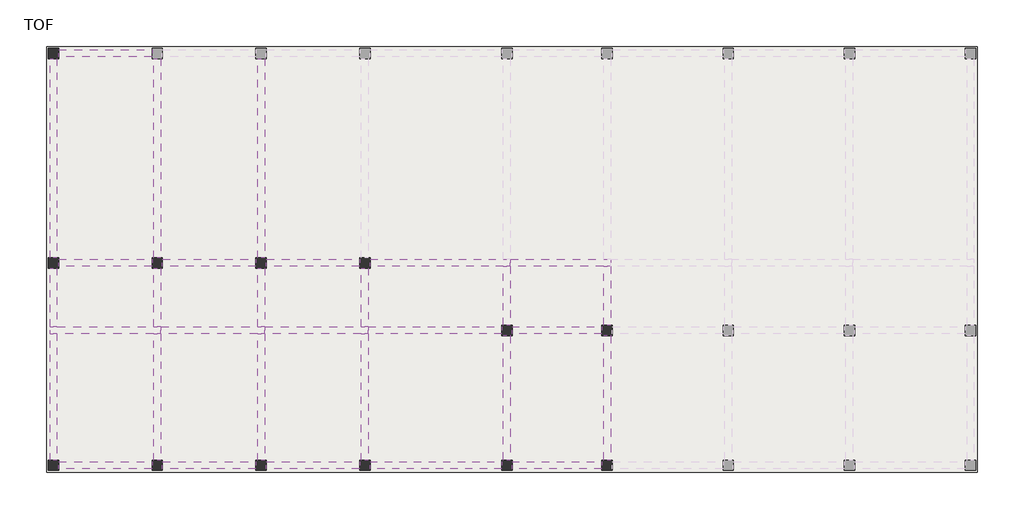
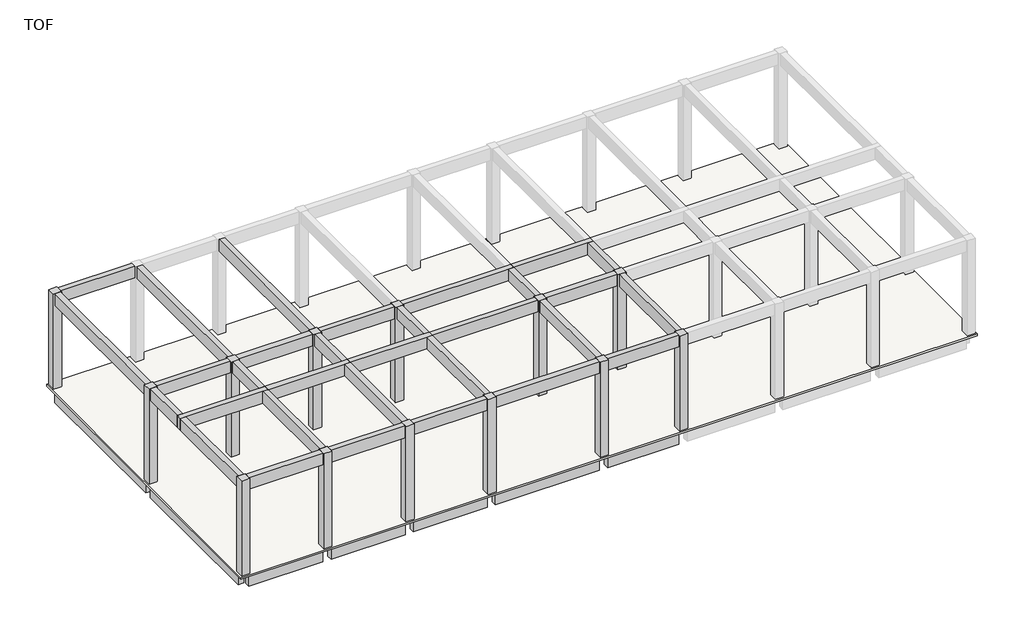
# One storey, part 1 of 2: 39 beams, 13 columns, 1 slab.
"""IFC4 building model written with IfcOpenShell, lengths in millimetres."""

from ifc_helpers import new_model, si_unit, frame, origin, origin_with_axes, place, context, project, spatial, polyline, outline, extrude, faceted_brep, element, save

model = new_model("IFC4")

# Units and contexts
model_context = context("Model", 3, world=origin())
ifc_project = project(units=[si_unit("LENGTHUNIT", "METRE", prefix="MILLI")], contexts=[model_context])

# Site, building, storey
site = spatial("IfcSite", under=ifc_project)
building = spatial("IfcBuilding", under=site)
storey = spatial("IfcBuildingStorey", under=building, Name="TOF", Elevation=150.0)

# Beams
placement = place(None, origin())
element("IfcBeam", 1, ObjectType="RC Beam_Rectangular : H_SB_ACB_B400xH900", at=placement, inside=storey, context=model_context, shape_type="SweptSolid", body=[
    extrude(outline(polyline([(124.7, 12616.5208589), (-275.3, 12616.5208589), (-275.3, 24116.5208589), (124.7, 24116.5208589), (124.7, 12616.5208589)])), frame((0.0, 0.0, -900.0), z_axis=(0.0, 0.0, 1.0), x_axis=(1.0, 0.0, 0.0)), (0.0, 0.0, 1.0), 900.0),
])
element("IfcBeam", 2, ObjectType="RC Beam_Rectangular : H_SB_ACB_B400xH900", at=placement, inside=storey, context=model_context, shape_type="SweptSolid", body=[
    extrude(outline(polyline([(124.7, 916.5208589), (-275.3, 916.5208589), (-275.3, 12016.5208589), (124.7, 12016.5208589), (124.7, 916.5208589)])), frame((0.0, 0.0, -900.0), z_axis=(0.0, 0.0, 1.0), x_axis=(1.0, 0.0, 0.0)), (0.0, 0.0, 1.0), 900.0),
])
element("IfcBeam", 3, ObjectType="RC Beam_Rectangular : H_SB_ACB_B400xH900", at=placement, inside=storey, context=model_context, shape_type="SweptSolid", body=[
    extrude(outline(polyline([(5624.7, 24616.5208589), (5624.7, 24216.5208589), (224.7, 24216.5208589), (224.7, 24616.5208589), (5624.7, 24616.5208589)])), frame((0.0, 0.0, -900.0), z_axis=(0.0, 0.0, 1.0), x_axis=(1.0, 0.0, 0.0)), (0.0, 0.0, 1.0), 900.0),
])
element("IfcBeam", 4, ObjectType="RC Beam_Rectangular : H_SB_ACB_B400xH900", at=placement, inside=storey, context=model_context, shape_type="SweptSolid", body=[
    extrude(outline(polyline([(224.7, 416.5208589), (224.7, 816.5208589), (5624.7, 816.5208589), (5624.7, 416.5208589), (224.7, 416.5208589)])), frame((0.0, 0.0, -900.0), z_axis=(0.0, 0.0, 1.0), x_axis=(1.0, 0.0, 0.0)), (0.0, 0.0, 1.0), 900.0),
])
element("IfcBeam", 5, ObjectType="RC Beam_Rectangular : H_SB_ACB_B400xH900", at=placement, inside=storey, context=model_context, shape_type="SweptSolid", body=[
    extrude(outline(polyline([(6224.7, 416.5208589), (6224.7, 816.5208589), (11624.7, 816.5208589), (11624.7, 416.5208589), (6224.7, 416.5208589)])), frame((0.0, 0.0, -900.0), z_axis=(0.0, 0.0, 1.0), x_axis=(1.0, 0.0, 0.0)), (0.0, 0.0, 1.0), 900.0),
])
element("IfcBeam", 6, ObjectType="RC Beam_Rectangular : H_SB_ACB_B400xH900", at=placement, inside=storey, context=model_context, shape_type="SweptSolid", body=[
    extrude(outline(polyline([(12224.7, 416.5208589), (12224.7, 816.5208589), (17624.7, 816.5208589), (17624.7, 416.5208589), (12224.7, 416.5208589)])), frame((0.0, 0.0, -900.0), z_axis=(0.0, 0.0, 1.0), x_axis=(1.0, 0.0, 0.0)), (0.0, 0.0, 1.0), 900.0),
])
element("IfcBeam", 7, ObjectType="RC Beam_Rectangular : H_SB_ACB_B400xH900", at=placement, inside=storey, context=model_context, shape_type="SweptSolid", body=[
    extrude(outline(polyline([(18224.7, 416.5208589), (18224.7, 816.5208589), (25824.7, 816.5208589), (25824.7, 416.5208589), (18224.7, 416.5208589)])), frame((0.0, 0.0, -900.0), z_axis=(0.0, 0.0, 1.0), x_axis=(1.0, 0.0, 0.0)), (0.0, 0.0, 1.0), 900.0),
])
element("IfcBeam", 8, ObjectType="RC Beam_Rectangular : H_SB_ACB_B400xH900", at=placement, inside=storey, context=model_context, shape_type="SweptSolid", body=[
    extrude(outline(polyline([(26424.7, 416.5208589), (26424.7, 816.5208589), (31624.7, 816.5208589), (31624.7, 416.5208589), (26424.7, 416.5208589)])), frame((0.0, 0.0, -900.0), z_axis=(0.0, 0.0, 1.0), x_axis=(1.0, 0.0, 0.0)), (0.0, 0.0, 1.0), 900.0),
])
element("IfcBeam", 9, ObjectType="RC Beam_Rectangular : H_SB_ACB_B400xH900", at=placement, inside=storey, context=model_context, shape_type="SweptSolid", body=[
    extrude(outline(polyline([(224.7, 12116.5208589), (224.7, 12516.5208589), (5624.7, 12516.5208589), (5624.7, 12116.5208589), (224.7, 12116.5208589)])), frame((0.0, 0.0, 6600.0), z_axis=(0.0, 0.0, 1.0), x_axis=(1.0, 0.0, 0.0)), (0.0, 0.0, 1.0), 900.0),
])
element("IfcBeam", 10, ObjectType="RC Beam_Rectangular : H_SB_ACB_B400xH900", at=placement, inside=storey, context=model_context, shape_type="SweptSolid", body=[
    extrude(outline(polyline([(6224.7, 12116.5208589), (6224.7, 12516.5208589), (11624.7, 12516.5208589), (11624.7, 12116.5208589), (6224.7, 12116.5208589)])), frame((0.0, 0.0, 6600.0), z_axis=(0.0, 0.0, 1.0), x_axis=(1.0, 0.0, 0.0)), (0.0, 0.0, 1.0), 900.0),
])
element("IfcBeam", 11, ObjectType="RC Beam_Rectangular : H_SB_ACB_B400xH900", at=placement, inside=storey, context=model_context, shape_type="SweptSolid", body=[
    extrude(outline(polyline([(12224.7, 12116.5208589), (12224.7, 12516.5208589), (17624.7, 12516.5208589), (17624.7, 12116.5208589), (12224.7, 12116.5208589)])), frame((0.0, 0.0, 6600.0), z_axis=(0.0, 0.0, 1.0), x_axis=(1.0, 0.0, 0.0)), (0.0, 0.0, 1.0), 900.0),
])
element("IfcBeam", 12, ObjectType="RC Beam_Rectangular : H_SB_ACB_B400xH900", at=placement, inside=storey, context=model_context, shape_type="Brep", body=[
    faceted_brep([(26324.7, 12116.5208589, 7500.0), (26324.7, 12516.5208589, 7500.0), (25924.7, 12516.5208589, 7500.0), (18224.7, 12516.5208589, 7500.0), (18224.7, 12116.5208589, 7500.0), (25924.7, 12116.5208589, 7500.0), (26324.7, 12116.5208589, 6600.0), (18224.7, 12116.5208589, 6600.0), (25924.7, 12116.5208589, 6600.0), (26324.7, 12516.5208589, 6600.0), (18224.7, 12516.5208589, 6600.0), (25924.7, 12516.5208589, 6600.0)], [[[0, 1, 2, 3, 4, 5]], [[6, 0, 5, 4, 7, 8]], [[9, 6, 8, 7, 10, 11]], [[1, 9, 11, 10, 3, 2]], [[4, 3, 10, 7]], [[1, 0, 6, 9]]]),
])
element("IfcBeam", 13, ObjectType="RC Beam_Rectangular : H_SB_ACB_B400xH900", at=placement, inside=storey, context=model_context, shape_type="Brep", body=[
    faceted_brep([(32124.7, 12116.5208589, 7500.0), (32124.7, 12516.5208589, 7500.0), (31724.7, 12516.5208589, 7500.0), (26324.7, 12516.5208589, 7500.0), (26324.7, 12116.5208589, 7500.0), (31724.7, 12116.5208589, 7500.0), (32124.7, 12116.5208589, 6600.0), (26324.7, 12116.5208589, 6600.0), (31724.7, 12116.5208589, 6600.0), (32124.7, 12516.5208589, 6600.0), (26324.7, 12516.5208589, 6600.0), (31724.7, 12516.5208589, 6600.0)], [[[0, 1, 2, 3, 4, 5]], [[6, 0, 5, 4, 7, 8]], [[9, 6, 8, 7, 10, 11]], [[1, 9, 11, 10, 3, 2]], [[1, 0, 6, 9]], [[4, 3, 10, 7]]]),
])
element("IfcBeam", 14, ObjectType="RC Beam_Rectangular : H_SB_ACB_B400xH900", at=placement, inside=storey, context=model_context, shape_type="SweptSolid", body=[
    extrude(outline(polyline([(224.7, 24216.5208589), (224.7, 24616.5208589), (5624.7, 24616.5208589), (5624.7, 24216.5208589), (224.7, 24216.5208589)])), frame((0.0, 0.0, 6600.0), z_axis=(0.0, 0.0, 1.0), x_axis=(1.0, 0.0, 0.0)), (0.0, 0.0, 1.0), 900.0),
])
element("IfcBeam", 15, ObjectType="RC Beam_Rectangular : H_SB_ACB_B400xH900", at=placement, inside=storey, context=model_context, shape_type="Brep", body=[
    faceted_brep([(-275.3, 8616.5208589, 7500.0), (-275.3, 8216.5208589, 7500.0), (124.7, 8216.5208589, 7500.0), (5724.7, 8216.5208589, 7500.0), (6124.7, 8216.5208589, 7500.0), (6124.7, 8616.5208589, 7500.0), (5724.7, 8616.5208589, 7500.0), (124.7, 8616.5208589, 7500.0), (-275.3, 8216.5208589, 6600.0), (124.7, 8216.5208589, 6600.0), (5724.7, 8216.5208589, 6600.0), (6124.7, 8216.5208589, 6600.0), (-275.3, 8616.5208589, 6600.0), (124.7, 8616.5208589, 6600.0), (5724.7, 8616.5208589, 6600.0), (6124.7, 8616.5208589, 6600.0)], [[[0, 1, 2, 3, 4, 5, 6, 7]], [[1, 8, 9, 10, 11, 4, 3, 2]], [[8, 12, 13, 14, 15, 11, 10, 9]], [[12, 0, 7, 6, 5, 15, 14, 13]], [[1, 0, 12, 8]], [[5, 4, 11, 15]]]),
])
element("IfcBeam", 16, ObjectType="RC Beam_Rectangular : H_SB_ACB_B400xH900", at=placement, inside=storey, context=model_context, shape_type="Brep", body=[
    faceted_brep([(12124.7, 8216.5208589, 7500.0), (12124.7, 8616.5208589, 7500.0), (11724.7, 8616.5208589, 7500.0), (6124.7, 8616.5208589, 7500.0), (6124.7, 8216.5208589, 7500.0), (11724.7, 8216.5208589, 7500.0), (12124.7, 8216.5208589, 6600.0), (6124.7, 8216.5208589, 6600.0), (11724.7, 8216.5208589, 6600.0), (12124.7, 8616.5208589, 6600.0), (6124.7, 8616.5208589, 6600.0), (11724.7, 8616.5208589, 6600.0)], [[[0, 1, 2, 3, 4, 5]], [[6, 0, 5, 4, 7, 8]], [[9, 6, 8, 7, 10, 11]], [[1, 9, 11, 10, 3, 2]], [[1, 0, 6, 9]], [[4, 3, 10, 7]]]),
])
element("IfcBeam", 17, ObjectType="RC Beam_Rectangular : H_SB_ACB_B400xH900", at=placement, inside=storey, context=model_context, shape_type="Brep", body=[
    faceted_brep([(18124.7, 8216.5208589, 7500.0), (18124.7, 8616.5208589, 7500.0), (17724.7, 8616.5208589, 7500.0), (12124.7, 8616.5208589, 7500.0), (12124.7, 8216.5208589, 7500.0), (17724.7, 8216.5208589, 7500.0), (18124.7, 8216.5208589, 6600.0), (12124.7, 8216.5208589, 6600.0), (17724.7, 8216.5208589, 6600.0), (18124.7, 8616.5208589, 6600.0), (12124.7, 8616.5208589, 6600.0), (17724.7, 8616.5208589, 6600.0)], [[[0, 1, 2, 3, 4, 5]], [[6, 0, 5, 4, 7, 8]], [[9, 6, 8, 7, 10, 11]], [[1, 9, 11, 10, 3, 2]], [[1, 0, 6, 9]], [[4, 3, 10, 7]]]),
])
element("IfcBeam", 18, ObjectType="RC Beam_Rectangular : H_SB_ACB_B400xH900", at=placement, inside=storey, context=model_context, shape_type="SweptSolid", body=[
    extrude(outline(polyline([(18124.7, 8216.5208589), (18124.7, 8616.5208589), (25824.7, 8616.5208589), (25824.7, 8216.5208589), (18124.7, 8216.5208589)])), frame((0.0, 0.0, 6600.0), z_axis=(0.0, 0.0, 1.0), x_axis=(1.0, 0.0, 0.0)), (0.0, 0.0, 1.0), 900.0),
])
element("IfcBeam", 19, ObjectType="RC Beam_Rectangular : H_SB_ACB_B400xH900", at=placement, inside=storey, context=model_context, shape_type="SweptSolid", body=[
    extrude(outline(polyline([(26424.7, 8216.5208589), (26424.7, 8616.5208589), (31624.7, 8616.5208589), (31624.7, 8216.5208589), (26424.7, 8216.5208589)])), frame((0.0, 0.0, 6600.0), z_axis=(0.0, 0.0, 1.0), x_axis=(1.0, 0.0, 0.0)), (0.0, 0.0, 1.0), 900.0),
])
element("IfcBeam", 20, ObjectType="RC Beam_Rectangular : H_SB_ACB_B400xH900", at=placement, inside=storey, context=model_context, shape_type="SweptSolid", body=[
    extrude(outline(polyline([(224.7, 416.5208589), (224.7, 816.5208589), (5624.7, 816.5208589), (5624.7, 416.5208589), (224.7, 416.5208589)])), frame((0.0, 0.0, 6600.0), z_axis=(0.0, 0.0, 1.0), x_axis=(1.0, 0.0, 0.0)), (0.0, 0.0, 1.0), 900.0),
])
element("IfcBeam", 21, ObjectType="RC Beam_Rectangular : H_SB_ACB_B400xH900", at=placement, inside=storey, context=model_context, shape_type="SweptSolid", body=[
    extrude(outline(polyline([(6224.7, 416.5208589), (6224.7, 816.5208589), (11624.7, 816.5208589), (11624.7, 416.5208589), (6224.7, 416.5208589)])), frame((0.0, 0.0, 6600.0), z_axis=(0.0, 0.0, 1.0), x_axis=(1.0, 0.0, 0.0)), (0.0, 0.0, 1.0), 900.0),
])
element("IfcBeam", 22, ObjectType="RC Beam_Rectangular : H_SB_ACB_B400xH900", at=placement, inside=storey, context=model_context, shape_type="SweptSolid", body=[
    extrude(outline(polyline([(12224.7, 416.5208589), (12224.7, 816.5208589), (17624.7, 816.5208589), (17624.7, 416.5208589), (12224.7, 416.5208589)])), frame((0.0, 0.0, 6600.0), z_axis=(0.0, 0.0, 1.0), x_axis=(1.0, 0.0, 0.0)), (0.0, 0.0, 1.0), 900.0),
])
element("IfcBeam", 23, ObjectType="RC Beam_Rectangular : H_SB_ACB_B400xH900", at=placement, inside=storey, context=model_context, shape_type="SweptSolid", body=[
    extrude(outline(polyline([(18224.7, 416.5208589), (18224.7, 816.5208589), (25824.7, 816.5208589), (25824.7, 416.5208589), (18224.7, 416.5208589)])), frame((0.0, 0.0, 6600.0), z_axis=(0.0, 0.0, 1.0), x_axis=(1.0, 0.0, 0.0)), (0.0, 0.0, 1.0), 900.0),
])
element("IfcBeam", 24, ObjectType="RC Beam_Rectangular : H_SB_ACB_B400xH900", at=placement, inside=storey, context=model_context, shape_type="SweptSolid", body=[
    extrude(outline(polyline([(26424.7, 416.5208589), (26424.7, 816.5208589), (31624.7, 816.5208589), (31624.7, 416.5208589), (26424.7, 416.5208589)])), frame((0.0, 0.0, 6600.0), z_axis=(0.0, 0.0, 1.0), x_axis=(1.0, 0.0, 0.0)), (0.0, 0.0, 1.0), 900.0),
])
element("IfcBeam", 25, ObjectType="RC Beam_Rectangular : H_SB_ACB_B400xH900", at=placement, inside=storey, context=model_context, shape_type="SweptSolid", body=[
    extrude(outline(polyline([(-275.3, 8216.5208589), (124.7, 8216.5208589), (124.7, 916.5208589), (-275.3, 916.5208589), (-275.3, 8216.5208589)])), frame((0.0, 0.0, 6600.0), z_axis=(0.0, 0.0, 1.0), x_axis=(1.0, 0.0, 0.0)), (0.0, 0.0, 1.0), 900.0),
])
element("IfcBeam", 26, ObjectType="RC Beam_Rectangular : H_SB_ACB_B400xH900", at=placement, inside=storey, context=model_context, shape_type="SweptSolid", body=[
    extrude(outline(polyline([(124.7, 8616.5208589), (-275.3, 8616.5208589), (-275.3, 12016.5208589), (124.7, 12016.5208589), (124.7, 8616.5208589)])), frame((0.0, 0.0, 6600.0), z_axis=(0.0, 0.0, 1.0), x_axis=(1.0, 0.0, 0.0)), (0.0, 0.0, 1.0), 900.0),
])
element("IfcBeam", 27, ObjectType="RC Beam_Rectangular : H_SB_ACB_B400xH900", at=placement, inside=storey, context=model_context, shape_type="SweptSolid", body=[
    extrude(outline(polyline([(124.7, 12616.5208589), (-275.3, 12616.5208589), (-275.3, 24116.5208589), (124.7, 24116.5208589), (124.7, 12616.5208589)])), frame((0.0, 0.0, 6600.0), z_axis=(0.0, 0.0, 1.0), x_axis=(1.0, 0.0, 0.0)), (0.0, 0.0, 1.0), 900.0),
])
element("IfcBeam", 28, ObjectType="RC Beam_Rectangular : H_SB_ACB_B400xH900", at=placement, inside=storey, context=model_context, shape_type="SweptSolid", body=[
    extrude(outline(polyline([(5724.7, 8216.5208589), (6124.7, 8216.5208589), (6124.7, 916.5208589), (5724.7, 916.5208589), (5724.7, 8216.5208589)])), frame((0.0, 0.0, 6600.0), z_axis=(0.0, 0.0, 1.0), x_axis=(1.0, 0.0, 0.0)), (0.0, 0.0, 1.0), 900.0),
])
element("IfcBeam", 29, ObjectType="RC Beam_Rectangular : H_SB_ACB_B400xH900", at=placement, inside=storey, context=model_context, shape_type="SweptSolid", body=[
    extrude(outline(polyline([(6124.7, 8616.5208589), (5724.7, 8616.5208589), (5724.7, 12016.5208589), (6124.7, 12016.5208589), (6124.7, 8616.5208589)])), frame((0.0, 0.0, 6600.0), z_axis=(0.0, 0.0, 1.0), x_axis=(1.0, 0.0, 0.0)), (0.0, 0.0, 1.0), 900.0),
])
element("IfcBeam", 30, ObjectType="RC Beam_Rectangular : H_SB_ACB_B400xH900", at=placement, inside=storey, context=model_context, shape_type="SweptSolid", body=[
    extrude(outline(polyline([(6124.7, 12616.5208589), (5724.7, 12616.5208589), (5724.7, 24116.5208589), (6124.7, 24116.5208589), (6124.7, 12616.5208589)])), frame((0.0, 0.0, 6600.0), z_axis=(0.0, 0.0, 1.0), x_axis=(1.0, 0.0, 0.0)), (0.0, 0.0, 1.0), 900.0),
])
element("IfcBeam", 31, ObjectType="RC Beam_Rectangular : H_SB_ACB_B400xH900", at=placement, inside=storey, context=model_context, shape_type="SweptSolid", body=[
    extrude(outline(polyline([(11724.7, 8216.5208589), (12124.7, 8216.5208589), (12124.7, 916.5208589), (11724.7, 916.5208589), (11724.7, 8216.5208589)])), frame((0.0, 0.0, 6600.0), z_axis=(0.0, 0.0, 1.0), x_axis=(1.0, 0.0, 0.0)), (0.0, 0.0, 1.0), 900.0),
])
element("IfcBeam", 32, ObjectType="RC Beam_Rectangular : H_SB_ACB_B400xH900", at=placement, inside=storey, context=model_context, shape_type="SweptSolid", body=[
    extrude(outline(polyline([(12124.7, 8616.5208589), (11724.7, 8616.5208589), (11724.7, 12016.5208589), (12124.7, 12016.5208589), (12124.7, 8616.5208589)])), frame((0.0, 0.0, 6600.0), z_axis=(0.0, 0.0, 1.0), x_axis=(1.0, 0.0, 0.0)), (0.0, 0.0, 1.0), 900.0),
])
element("IfcBeam", 33, ObjectType="RC Beam_Rectangular : H_SB_ACB_B400xH900", at=placement, inside=storey, context=model_context, shape_type="SweptSolid", body=[
    extrude(outline(polyline([(12124.7, 12616.5208589), (11724.7, 12616.5208589), (11724.7, 24116.5208589), (12124.7, 24116.5208589), (12124.7, 12616.5208589)])), frame((0.0, 0.0, 6600.0), z_axis=(0.0, 0.0, 1.0), x_axis=(1.0, 0.0, 0.0)), (0.0, 0.0, 1.0), 900.0),
])
element("IfcBeam", 34, ObjectType="RC Beam_Rectangular : H_SB_ACB_B400xH900", at=placement, inside=storey, context=model_context, shape_type="SweptSolid", body=[
    extrude(outline(polyline([(17724.7, 8216.5208589), (18124.7, 8216.5208589), (18124.7, 916.5208589), (17724.7, 916.5208589), (17724.7, 8216.5208589)])), frame((0.0, 0.0, 6600.0), z_axis=(0.0, 0.0, 1.0), x_axis=(1.0, 0.0, 0.0)), (0.0, 0.0, 1.0), 900.0),
])
element("IfcBeam", 35, ObjectType="RC Beam_Rectangular : H_SB_ACB_B400xH900", at=placement, inside=storey, context=model_context, shape_type="SweptSolid", body=[
    extrude(outline(polyline([(18124.7, 8616.5208589), (17724.7, 8616.5208589), (17724.7, 12016.5208589), (18124.7, 12016.5208589), (18124.7, 8616.5208589)])), frame((0.0, 0.0, 6600.0), z_axis=(0.0, 0.0, 1.0), x_axis=(1.0, 0.0, 0.0)), (0.0, 0.0, 1.0), 900.0),
])
element("IfcBeam", 36, ObjectType="RC Beam_Rectangular : H_SB_ACB_B400xH900", at=placement, inside=storey, context=model_context, shape_type="SweptSolid", body=[
    extrude(outline(polyline([(25924.7, 8116.5208589), (26324.7, 8116.5208589), (26324.7, 916.5208589), (25924.7, 916.5208589), (25924.7, 8116.5208589)])), frame((0.0, 0.0, 6600.0), z_axis=(0.0, 0.0, 1.0), x_axis=(1.0, 0.0, 0.0)), (0.0, 0.0, 1.0), 900.0),
])
element("IfcBeam", 37, ObjectType="RC Beam_Rectangular : H_SB_ACB_B400xH900", at=placement, inside=storey, context=model_context, shape_type="SweptSolid", body=[
    extrude(outline(polyline([(25924.7, 12116.5208589), (26324.7, 12116.5208589), (26324.7, 8716.5208589), (25924.7, 8716.5208589), (25924.7, 12116.5208589)])), frame((0.0, 0.0, 6600.0), z_axis=(0.0, 0.0, 1.0), x_axis=(1.0, 0.0, 0.0)), (0.0, 0.0, 1.0), 900.0),
])
element("IfcBeam", 38, ObjectType="RC Beam_Rectangular : H_SB_ACB_B400xH900", at=placement, inside=storey, context=model_context, shape_type="SweptSolid", body=[
    extrude(outline(polyline([(31724.7, 8116.5208589), (32124.7, 8116.5208589), (32124.7, 916.5208589), (31724.7, 916.5208589), (31724.7, 8116.5208589)])), frame((0.0, 0.0, 6600.0), z_axis=(0.0, 0.0, 1.0), x_axis=(1.0, 0.0, 0.0)), (0.0, 0.0, 1.0), 900.0),
])
element("IfcBeam", 39, ObjectType="RC Beam_Rectangular : H_SB_ACB_B400xH900", at=placement, inside=storey, context=model_context, shape_type="SweptSolid", body=[
    extrude(outline(polyline([(31724.7, 12116.5208589), (32124.7, 12116.5208589), (32124.7, 8716.5208589), (31724.7, 8716.5208589), (31724.7, 12116.5208589)])), frame((0.0, 0.0, 6600.0), z_axis=(0.0, 0.0, 1.0), x_axis=(1.0, 0.0, 0.0)), (0.0, 0.0, 1.0), 900.0),
])

# Columns
element("IfcColumn", 40, ObjectType="RC_Column_Rectangular : H_SC_ACC_W600xL600", at=placement, inside=storey, context=model_context, shape_type="Brep", body=[
    faceted_brep([(224.7, 12616.5208589, 7500.0), (224.7, 12516.5208589, 7500.0), (224.7, 12116.5208589, 7500.0), (224.7, 12016.5208589, 7500.0), (224.7, 12016.5208589, 150.0), (224.7, 12616.5208589, 150.0), (124.7, 12016.5208589, 7500.0), (-275.3, 12016.5208589, 7500.0), (-375.3, 12016.5208589, 7500.0), (-375.3, 12016.5208589, 150.0), (-375.3, 12616.5208589, 7500.0), (-375.3, 12616.5208589, 150.0), (-275.3, 12616.5208589, 7500.0), (124.7, 12616.5208589, 7500.0)], [[[0, 1, 2, 3, 4, 5]], [[3, 6, 7, 8, 9, 4]], [[8, 10, 11, 9]], [[10, 12, 13, 0, 5, 11]], [[3, 2, 1, 0, 13, 12, 10, 8, 7, 6]], [[5, 4, 9, 11]]]),
])
element("IfcColumn", 41, ObjectType="RC_Column_Rectangular : H_SC_ACC_W600xL600", at=placement, inside=storey, context=model_context, shape_type="Brep", body=[
    faceted_brep([(6224.7, 12616.5208589, 7500.0), (6224.7, 12516.5208589, 7500.0), (6224.7, 12116.5208589, 7500.0), (6224.7, 12016.5208589, 7500.0), (6224.7, 12016.5208589, 150.0), (6224.7, 12616.5208589, 150.0), (6124.7, 12016.5208589, 7500.0), (5724.7, 12016.5208589, 7500.0), (5624.7, 12016.5208589, 7500.0), (5624.7, 12016.5208589, 150.0), (5624.7, 12116.5208589, 7500.0), (5624.7, 12516.5208589, 7500.0), (5624.7, 12616.5208589, 7500.0), (5624.7, 12616.5208589, 150.0), (5724.7, 12616.5208589, 7500.0), (6124.7, 12616.5208589, 7500.0)], [[[0, 1, 2, 3, 4, 5]], [[3, 6, 7, 8, 9, 4]], [[8, 10, 11, 12, 13, 9]], [[12, 14, 15, 0, 5, 13]], [[3, 2, 1, 0, 15, 14, 12, 11, 10, 8, 7, 6]], [[5, 4, 9, 13]]]),
])
element("IfcColumn", 42, ObjectType="RC_Column_Rectangular : H_SC_ACC_W600xL600", at=placement, inside=storey, context=model_context, shape_type="Brep", body=[
    faceted_brep([(12224.7, 12616.5208589, 7500.0), (12224.7, 12516.5208589, 7500.0), (12224.7, 12116.5208589, 7500.0), (12224.7, 12016.5208589, 7500.0), (12224.7, 12016.5208589, 150.0), (12224.7, 12616.5208589, 150.0), (12124.7, 12016.5208589, 7500.0), (11724.7, 12016.5208589, 7500.0), (11624.7, 12016.5208589, 7500.0), (11624.7, 12016.5208589, 150.0), (11624.7, 12116.5208589, 7500.0), (11624.7, 12516.5208589, 7500.0), (11624.7, 12616.5208589, 7500.0), (11624.7, 12616.5208589, 150.0), (11724.7, 12616.5208589, 7500.0), (12124.7, 12616.5208589, 7500.0)], [[[0, 1, 2, 3, 4, 5]], [[3, 6, 7, 8, 9, 4]], [[8, 10, 11, 12, 13, 9]], [[12, 14, 15, 0, 5, 13]], [[3, 2, 1, 0, 15, 14, 12, 11, 10, 8, 7, 6]], [[5, 4, 9, 13]]]),
])
element("IfcColumn", 43, ObjectType="RC_Column_Rectangular : H_SC_ACC_W600xL600", at=placement, inside=storey, context=model_context, shape_type="Brep", body=[
    faceted_brep([(18224.7, 12616.5208589, 7500.0), (18224.7, 12516.5208589, 7500.0), (18224.7, 12116.5208589, 7500.0), (18224.7, 12016.5208589, 7500.0), (18224.7, 12016.5208589, 150.0), (18224.7, 12616.5208589, 150.0), (18124.7, 12016.5208589, 7500.0), (17724.7, 12016.5208589, 7500.0), (17624.7, 12016.5208589, 7500.0), (17624.7, 12016.5208589, 150.0), (17624.7, 12116.5208589, 7500.0), (17624.7, 12516.5208589, 7500.0), (17624.7, 12616.5208589, 7500.0), (17624.7, 12616.5208589, 150.0), (17724.7, 12616.5208589, 7500.0), (18124.7, 12616.5208589, 7500.0)], [[[0, 1, 2, 3, 4, 5]], [[3, 6, 7, 8, 9, 4]], [[8, 10, 11, 12, 13, 9]], [[12, 14, 15, 0, 5, 13]], [[3, 2, 1, 0, 15, 14, 12, 11, 10, 8, 7, 6]], [[5, 4, 9, 13]]]),
])
element("IfcColumn", 44, ObjectType="RC_Column_Rectangular : H_SC_ACC_W600xL600", at=placement, inside=storey, context=model_context, shape_type="Brep", body=[
    faceted_brep([(224.7, 24716.5208589, 7500.0), (224.7, 24616.5208589, 7500.0), (224.7, 24216.5208589, 7500.0), (224.7, 24116.5208589, 7500.0), (224.7, 24116.5208589, 150.0), (224.7, 24716.5208589, 150.0), (124.7, 24116.5208589, 7500.0), (-275.3, 24116.5208589, 7500.0), (-375.3, 24116.5208589, 7500.0), (-375.3, 24116.5208589, 150.0), (-375.3, 24716.5208589, 7500.0), (-375.3, 24716.5208589, 150.0)], [[[0, 1, 2, 3, 4, 5]], [[3, 6, 7, 8, 9, 4]], [[8, 10, 11, 9]], [[10, 0, 5, 11]], [[3, 2, 1, 0, 10, 8, 7, 6]], [[5, 4, 9, 11]]]),
])
element("IfcColumn", 45, ObjectType="RC_Column_Rectangular : H_SC_ACC_W600xL600", at=placement, inside=storey, context=model_context, shape_type="Brep", body=[
    faceted_brep([(26424.7, 8716.5208589, 7500.0), (26424.7, 8616.5208589, 7500.0), (26424.7, 8216.5208589, 7500.0), (26424.7, 8116.5208589, 7500.0), (26424.7, 8116.5208589, 150.0), (26424.7, 8716.5208589, 150.0), (26324.7, 8116.5208589, 7500.0), (25924.7, 8116.5208589, 7500.0), (25824.7, 8116.5208589, 7500.0), (25824.7, 8116.5208589, 150.0), (25824.7, 8216.5208589, 7500.0), (25824.7, 8616.5208589, 7500.0), (25824.7, 8716.5208589, 7500.0), (25824.7, 8716.5208589, 150.0), (25924.7, 8716.5208589, 7500.0), (26324.7, 8716.5208589, 7500.0)], [[[0, 1, 2, 3, 4, 5]], [[3, 6, 7, 8, 9, 4]], [[8, 10, 11, 12, 13, 9]], [[12, 14, 15, 0, 5, 13]], [[3, 2, 1, 0, 15, 14, 12, 11, 10, 8, 7, 6]], [[5, 4, 9, 13]]]),
])
element("IfcColumn", 46, ObjectType="RC_Column_Rectangular : H_SC_ACC_W600xL600", at=placement, inside=storey, context=model_context, shape_type="Brep", body=[
    faceted_brep([(32224.7, 8716.5208589, 7500.0), (32224.7, 8616.5208589, 7500.0), (32224.7, 8216.5208589, 7500.0), (32224.7, 8116.5208589, 7500.0), (32224.7, 8116.5208589, 150.0), (32224.7, 8716.5208589, 150.0), (32124.7, 8116.5208589, 7500.0), (31724.7, 8116.5208589, 7500.0), (31624.7, 8116.5208589, 7500.0), (31624.7, 8116.5208589, 150.0), (31624.7, 8216.5208589, 7500.0), (31624.7, 8616.5208589, 7500.0), (31624.7, 8716.5208589, 7500.0), (31624.7, 8716.5208589, 150.0), (31724.7, 8716.5208589, 7500.0), (32124.7, 8716.5208589, 7500.0)], [[[0, 1, 2, 3, 4, 5]], [[3, 6, 7, 8, 9, 4]], [[8, 10, 11, 12, 13, 9]], [[12, 14, 15, 0, 5, 13]], [[3, 2, 1, 0, 15, 14, 12, 11, 10, 8, 7, 6]], [[5, 4, 9, 13]]]),
])
element("IfcColumn", 47, ObjectType="RC_Column_Rectangular : H_SC_ACC_W600xL600", at=placement, inside=storey, context=model_context, shape_type="Brep", body=[
    faceted_brep([(224.7, 916.5208589, 7500.0), (224.7, 816.5208589, 7500.0), (224.7, 416.5208589, 7500.0), (224.7, 316.5208589, 7500.0), (224.7, 316.5208589, 150.0), (224.7, 916.5208589, 150.0), (-375.3, 316.5208589, 7500.0), (-375.3, 316.5208589, 150.0), (-375.3, 916.5208589, 7500.0), (-375.3, 916.5208589, 150.0), (-275.3, 916.5208589, 7500.0), (124.7, 916.5208589, 7500.0)], [[[0, 1, 2, 3, 4, 5]], [[3, 6, 7, 4]], [[6, 8, 9, 7]], [[8, 10, 11, 0, 5, 9]], [[3, 2, 1, 0, 11, 10, 8, 6]], [[5, 4, 7, 9]]]),
])
element("IfcColumn", 48, ObjectType="RC_Column_Rectangular : H_SC_ACC_W600xL600", at=placement, inside=storey, context=model_context, shape_type="Brep", body=[
    faceted_brep([(6224.7, 916.5208589, 7500.0), (6224.7, 816.5208589, 7500.0), (6224.7, 416.5208589, 7500.0), (6224.7, 316.5208589, 7500.0), (6224.7, 316.5208589, 150.0), (6224.7, 916.5208589, 150.0), (5624.7, 316.5208589, 7500.0), (5624.7, 316.5208589, 150.0), (5624.7, 416.5208589, 7500.0), (5624.7, 816.5208589, 7500.0), (5624.7, 916.5208589, 7500.0), (5624.7, 916.5208589, 150.0), (5724.7, 916.5208589, 7500.0), (6124.7, 916.5208589, 7500.0)], [[[0, 1, 2, 3, 4, 5]], [[3, 6, 7, 4]], [[6, 8, 9, 10, 11, 7]], [[10, 12, 13, 0, 5, 11]], [[3, 2, 1, 0, 13, 12, 10, 9, 8, 6]], [[5, 4, 7, 11]]]),
])
element("IfcColumn", 49, ObjectType="RC_Column_Rectangular : H_SC_ACC_W600xL600", at=placement, inside=storey, context=model_context, shape_type="Brep", body=[
    faceted_brep([(12224.7, 916.5208589, 7500.0), (12224.7, 816.5208589, 7500.0), (12224.7, 416.5208589, 7500.0), (12224.7, 316.5208589, 7500.0), (12224.7, 316.5208589, 150.0), (12224.7, 916.5208589, 150.0), (11624.7, 316.5208589, 7500.0), (11624.7, 316.5208589, 150.0), (11624.7, 416.5208589, 7500.0), (11624.7, 816.5208589, 7500.0), (11624.7, 916.5208589, 7500.0), (11624.7, 916.5208589, 150.0), (11724.7, 916.5208589, 7500.0), (12124.7, 916.5208589, 7500.0)], [[[0, 1, 2, 3, 4, 5]], [[3, 6, 7, 4]], [[6, 8, 9, 10, 11, 7]], [[10, 12, 13, 0, 5, 11]], [[3, 2, 1, 0, 13, 12, 10, 9, 8, 6]], [[5, 4, 7, 11]]]),
])
element("IfcColumn", 50, ObjectType="RC_Column_Rectangular : H_SC_ACC_W600xL600", at=placement, inside=storey, context=model_context, shape_type="Brep", body=[
    faceted_brep([(18224.7, 916.5208589, 7500.0), (18224.7, 816.5208589, 7500.0), (18224.7, 416.5208589, 7500.0), (18224.7, 316.5208589, 7500.0), (18224.7, 316.5208589, 150.0), (18224.7, 916.5208589, 150.0), (17624.7, 316.5208589, 7500.0), (17624.7, 316.5208589, 150.0), (17624.7, 416.5208589, 7500.0), (17624.7, 816.5208589, 7500.0), (17624.7, 916.5208589, 7500.0), (17624.7, 916.5208589, 150.0), (17724.7, 916.5208589, 7500.0), (18124.7, 916.5208589, 7500.0)], [[[0, 1, 2, 3, 4, 5]], [[3, 6, 7, 4]], [[6, 8, 9, 10, 11, 7]], [[10, 12, 13, 0, 5, 11]], [[3, 2, 1, 0, 13, 12, 10, 9, 8, 6]], [[5, 4, 7, 11]]]),
])
element("IfcColumn", 51, ObjectType="RC_Column_Rectangular : H_SC_ACC_W600xL600", at=placement, inside=storey, context=model_context, shape_type="Brep", body=[
    faceted_brep([(26424.7, 916.5208589, 7500.0), (26424.7, 816.5208589, 7500.0), (26424.7, 416.5208589, 7500.0), (26424.7, 316.5208589, 7500.0), (26424.7, 316.5208589, 150.0), (26424.7, 916.5208589, 150.0), (25824.7, 316.5208589, 7500.0), (25824.7, 316.5208589, 150.0), (25824.7, 416.5208589, 7500.0), (25824.7, 816.5208589, 7500.0), (25824.7, 916.5208589, 7500.0), (25824.7, 916.5208589, 150.0), (25924.7, 916.5208589, 7500.0), (26324.7, 916.5208589, 7500.0)], [[[0, 1, 2, 3, 4, 5]], [[3, 6, 7, 4]], [[6, 8, 9, 10, 11, 7]], [[10, 12, 13, 0, 5, 11]], [[3, 2, 1, 0, 13, 12, 10, 9, 8, 6]], [[5, 4, 7, 11]]]),
])
element("IfcColumn", 52, ObjectType="RC_Column_Rectangular : H_SC_ACC_W600xL600", at=placement, inside=storey, context=model_context, shape_type="Brep", body=[
    faceted_brep([(32224.7, 916.5208589, 7500.0), (32224.7, 816.5208589, 7500.0), (32224.7, 416.5208589, 7500.0), (32224.7, 316.5208589, 7500.0), (32224.7, 316.5208589, 150.0), (32224.7, 916.5208589, 150.0), (31624.7, 316.5208589, 7500.0), (31624.7, 316.5208589, 150.0), (31624.7, 416.5208589, 7500.0), (31624.7, 816.5208589, 7500.0), (31624.7, 916.5208589, 7500.0), (31624.7, 916.5208589, 150.0), (31724.7, 916.5208589, 7500.0), (32124.7, 916.5208589, 7500.0)], [[[0, 1, 2, 3, 4, 5]], [[3, 6, 7, 4]], [[6, 8, 9, 10, 11, 7]], [[10, 12, 13, 0, 5, 11]], [[3, 2, 1, 0, 13, 12, 10, 9, 8, 6]], [[5, 4, 7, 11]]]),
])

# Slab
element("IfcSlab", 53, ObjectType="H_FL_AMF_RC Slab_T150", at=placement, inside=storey, context=model_context, shape_type="SweptSolid", body=[
    extrude(outline(polyline([(53324.7, 216.5208589), (-475.3, 216.5208589), (-475.3, 24816.5208589), (53324.7, 24816.5208589), (53324.7, 216.5208589)])), origin_with_axes(), (0.0, 0.0, 1.0), 150.0),
])

save(model, "model.ifc")

# Revit data of these elements
# Project information
#   Project Status = "Project Status"
#   Client Name = "현대엔지니어링"
#   Project Address = "서울시 종로구 율곡로 75(계동)"
#   Project Number = "-"
# Grids (mm)
#   "Y1": line (-3935.398, 24416.521) -> (58968.688, 24416.521)
#   "X1": line (-75.3, 29394.337) -> (-75.3, -4379.638)
#   "X2": line (5924.7, 29394.337) -> (5924.7, -4379.638)
#   "Y3": line (-3935.398, 8416.521) -> (58968.688, 8416.521)
#   "Y4": line (-3935.398, 616.521) -> (58968.688, 616.521)
#   "X3": line (11924.7, 29394.337) -> (11924.7, -4379.638)
#   "X4": line (17924.7, 29394.337) -> (17924.7, -4379.638)
#   "X5": line (26124.7, 29394.337) -> (26124.7, -4379.638)
#   "X6": line (31924.7, 29394.337) -> (31924.7, -4379.638)
#   "X7": line (38924.7, 29394.337) -> (38924.7, -4379.638)
#   "X8": line (45924.7, 29394.337) -> (45924.7, -4379.638)
#   "X9": line (52924.7, 29394.337) -> (52924.7, -4379.638)
#   "X15": line (43724.7, 27041.858) -> (43724.7, 9156.488)
#   "X16": line (36324.7, 27041.858) -> (36324.7, 9156.488)
#   "X17": line (34685.051, 10966.521) -> (55094.626, 10966.521)
#   "X18": line (34685.051, 18666.521) -> (55094.626, 18666.521)
#   "Y2": line (-3935.398, 12316.521) -> (58968.688, 12316.521)
# Type "RC Beam_Rectangular : H_SB_ACB_B400xH900"
#   중앙부 하부근 = ""
#   중앙부 상부근 = ""
#   중앙부 보조근 = ""
#   중앙부 늑근 = ""
#   외단부 하부근 = ""
#   외단부 상부근 = ""
#   외단부 보조근 = ""
#   외단부 늑근 = ""
#   부호 = "TG3"
#   내단부 하부근 = ""
#   내단부 상부근 = ""
#   내단부 보조근 = ""
#   내단부 늑근 = ""
#   ALL 하부근 = "3-D20"
#   ALL 상부근 = "3-D20"
#   ALL 보조근 = ""
#   ALL 늑근 = "2-D10 @120"
#   Width = 400.000 mm
#   Height = 900.000 mm
#   Length [instance default] = 1524.000 mm
#   b = 400.000 mm
#   h = 900.000 mm
#   hec_material3 [instance default] = none
#   hec_material2 [instance default] = none
#   hec_material1 [instance default] = none
#   Structural Material [instance default] = none
#   Assembly Code = ""
# Type "RC_Column_Rectangular : H_SC_ACC_W600xL600"
#   Width = 600.000 mm
#   Length = 600.000 mm
#   hec_material3 [instance default] = none
#   hec_material2 [instance default] = none
#   hec_material1 [instance default] = none
#   Structural Material [instance default] = none
#   Description = (empty or 0)
# Type "H_FL_AMF_RC Slab_T150"
#   Keynote = ""
#   Type Comments = ""
#   Description = ""
#   Function = 1
#   Layers, outside or top first: 150.000 mm no material (function 1)
# Elements 1, 2, 3, 4, 5, 6, 7, 8, 9, 10, 11, 12, 13, 14, 15, 16, 17, 18, 19, 20, 21, 22, 23, 24, 25, 26, 27, 28, 29, 30, 31, 32, 33, 34, 35, 36, 37, 38, 39 (IfcBeam, "RC Beam_Rectangular : H_SB_ACB_B400xH900")
#   hec_material3 = none
#   hec_material2 = none
#   hec_material1 = none
#   Structural Material = none
#   Phase Created = New Construction
# Elements 40, 41, 42, 43, 44, 45, 46, 47, 48, 49, 50, 51, 52 (IfcColumn, "RC_Column_Rectangular : H_SC_ACC_W600xL600")
#   Comments = ""
#   hec_material3 = none
#   hec_material2 = none
#   hec_material1 = none
#   Structural Material = none
#   Phase Created = New Construction
# Element 53 (IfcSlab, "H_FL_AMF_RC Slab_T150")
#   Height Offset From Level = 0.000 mm
#   Phase Created = New Construction
#   Materials on its faces: "Default Floor"
# Materials
#   "Default Floor": class "Miscellaneous", colour RGB 80 80 80, transparency 0
